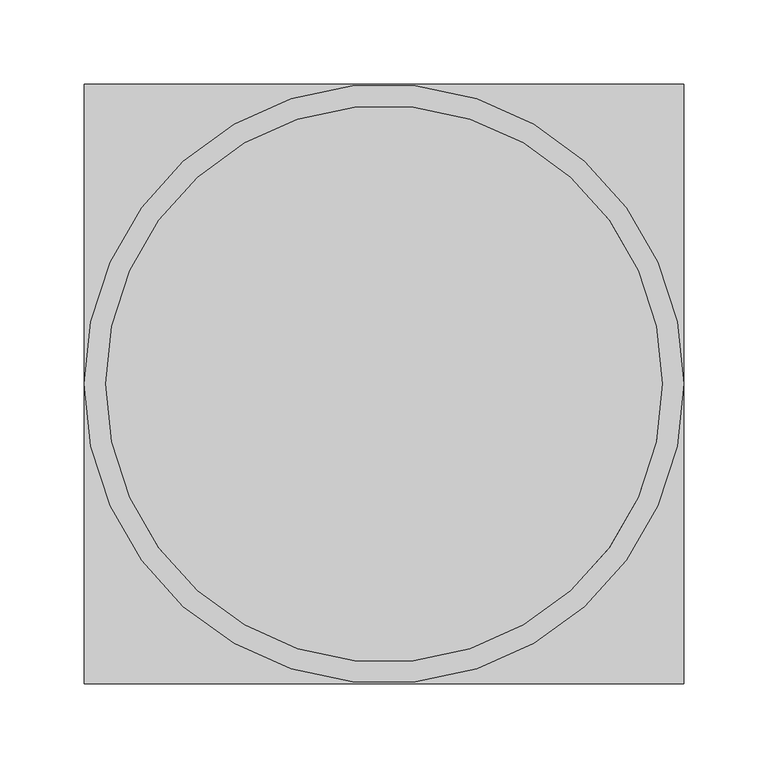
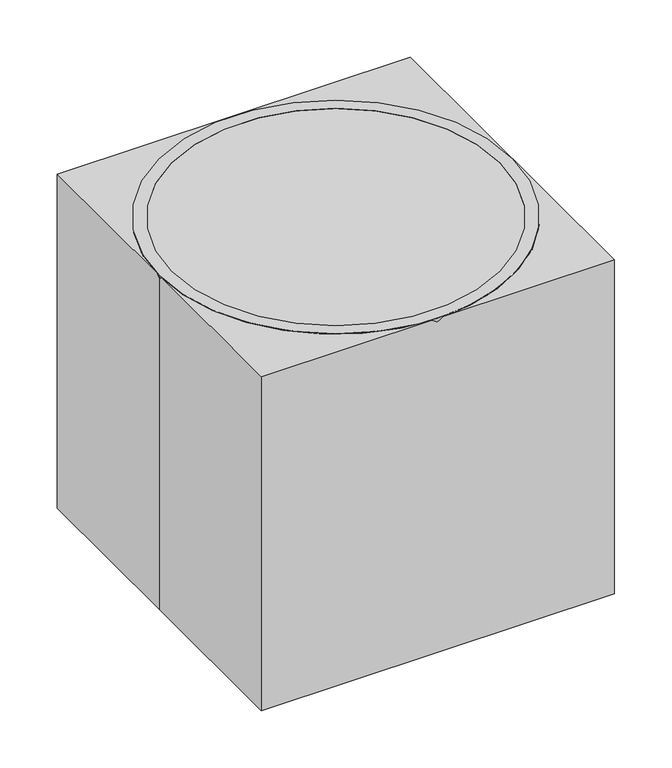
"""IFC4 building model written with IfcOpenShell, lengths in millimetres: proxy geometry, M8905 - Pail, Utility, CRS, Without Carriage : M8905 - Pail, Utility, CRS, Without Carriage."""

from ifc_helpers import new_model, si_unit, frame, origin, origin_with_axes, place, context, project, spatial, polyline, circle_curve, outline, extrude, source, transform, mapped, element, save
from ifc_brep_helpers import plane_surface, revolved_surface, advanced_brep


def specialty_equipment_c63f0c81(model_context):
    return source(origin(), model_context, "Body", "SolidModel", [
        advanced_brep(
        [(-127.0, 0.0, 0.0), (127.0, 0.0, 0.0), (-177.8, 0.0, 355.6), (177.8, 0.0, 355.6), (-165.1, 0.0, 355.6), (165.1, 0.0, 355.6), (114.3, 0.0, 19.5959229), (-114.3, 0.0, 19.5959229)],
        [
            (0, 1, circle_curve(frame((0.0, 0.0, 0.0), z_axis=(0.0, 0.0, -1.0), x_axis=(-1.0, 0.0, 0.0)), 127.0)),
            (1, 0, circle_curve(frame((0.0, 0.0, 0.0), z_axis=(0.0, 0.0, -1.0), x_axis=(1.0, 0.0, 0.0)), 127.0)),
            (2, 3, circle_curve(frame((0.0, 0.0, 355.6), z_axis=(0.0, 0.0, 1.0), x_axis=(1.0, 0.0, 0.0)), 177.8)),
            (3, 2, circle_curve(frame((0.0, 0.0, 355.6), z_axis=(0.0, 0.0, 1.0), x_axis=(-1.0, 0.0, 0.0)), 177.8)),
            (4, 5, circle_curve(frame((0.0, 0.0, 355.6), z_axis=(0.0, 0.0, -1.0), x_axis=(-1.0, 0.0, 0.0)), 165.1)),
            (5, 4, circle_curve(frame((0.0, 0.0, 355.6), z_axis=(0.0, 0.0, -1.0), x_axis=(1.0, 0.0, 0.0)), 165.1)),
            (1, 3),
            (2, 0),
            (6, 7, circle_curve(frame((0.0, 0.0, 19.5959229), z_axis=(0.0, 0.0, 1.0), x_axis=(-1.0, 0.0, 0.0)), 114.3)),
            (7, 6, circle_curve(frame((0.0, 0.0, 19.5959229), z_axis=(0.0, 0.0, 1.0), x_axis=(1.0, 0.0, 0.0)), 114.3)),
            (6, 5),
            (4, 7),
        ],
        [
            plane_surface(frame((0.0, 0.0, 0.0), z_axis=(0.0, 0.0, -1.0), x_axis=(0.0, -1.0, 0.0))),
            plane_surface(frame((0.0, 0.0, 355.6), z_axis=(0.0, 0.0, 1.0), x_axis=(0.0, -1.0, 0.0))),
            revolved_surface(polyline([(127.00000000000001, 0.0, 0.0), (177.8, 0.0, 355.5999999999999)]), (0.0, 0.0, -889.0), (0.0, 0.0, 1.0)),
            revolved_surface(polyline([(-127.00000000000001, 0.0, 0.0), (-177.8, 0.0, 355.5999999999999)]), (0.0, 0.0, -889.0), (0.0, 0.0, 1.0)),
            plane_surface(frame((0.0, 0.0, 19.5959229), z_axis=(0.0, 0.0, 1.0), x_axis=(0.0, -1.0, 0.0))),
            revolved_surface(polyline([(165.1, 0.0, 355.60000000000014), (114.299999996511, 0.0, 19.595922900000005)]), (0.0, 0.0, -736.4132505), (0.0, 0.0, 1.0)),
            revolved_surface(polyline([(-165.1, 0.0, 355.60000000000014), (-114.299999996511, 0.0, 19.595922900000005)]), (0.0, 0.0, -736.4132505), (0.0, 0.0, 1.0)),
        ],
        [
            (0, [[1, 2]]),
            (1, [[3, 4], [5, 6]]),
            (2, [[-2, 7, -3, 8]]),
            (3, [[-1, -8, -4, -7]]),
            (4, [[9, 10]]),
            (5, [[-9, 11, -5, 12]]),
            (6, [[-10, -12, -6, -11]]),
        ],
    ),
        extrude(outline(polyline([(-177.8, 177.8), (177.8, 177.8), (177.8, -177.8), (-177.8, -177.8), (-177.8, 0.0), (-177.8, 177.8)])), origin_with_axes(), (0.0, 0.0, 1.0), 355.6),
    ])


if __name__ == "__main__":
    model = new_model("IFC4")
    model_context = context("Model", 3, world=origin())
    ifc_project = project(units=[si_unit("LENGTHUNIT", "METRE", prefix="MILLI")], contexts=[model_context])
    site = spatial("IfcSite", under=ifc_project)
    building = spatial("IfcBuilding", under=site)
    placement = place(None, origin())
    specialty_equipment_shape = specialty_equipment_c63f0c81(model_context)
    element("IfcBuildingElementProxy", 1, Name="M8905 - Pail, Utility, CRS, Without Carriage : M8905 - Pail, Utility, CRS, Without Carriage", ObjectType="M8905 - Pail, Utility, CRS, Without Carriage : M8905 - Pail, Utility, CRS, Without Carriage", at=placement, inside=building, context=model_context, shape_type="MappedRepresentation", body=[
        mapped(specialty_equipment_shape, transform((0.0, 0.0, 0.0), x_axis=(1.0, 0.0, 0.0), y_axis=(0.0, 1.0, 0.0), z_axis=(0.0, 0.0, 1.0))),
    ])
    save(model, "model.ifc")

# Revit data of these elements
# Type "M8905 - Pail, Utility, CRS, Without Carriage : M8905 - Pail, Utility, CRS, Without Carriage"
#   Watts2 = "0"
#   Watts1 = "0"
#   Unit_Issue = "EA"
#   UTIL_6_Misc = "-"
#   UTIL_5_NonMedGas = "-"
#   UTIL_4_MiscGas = "-"
#   UTIL_3_MedGas = "-"
#   UTIL_2_Elec = "-"
#   UTIL_1_WaterDrain = "-"
#   Nomenclature = "Pail, Utility, CRS, Without Carriage"
#   NSN = "6530"
#   Location [instance default] = ""
#   JSN = "M8905"
#   Fund_Source_VA = "-"
#   Fund_Source_Navy = "-"
#   Fund_Source_Army = "-"
#   Fund_Source_AF = "-"
#   ELEC_Volts2 = "0"
#   ELEC_Volts1 = "0"
#   ELEC_Phase2 = "0"
#   ELEC_Phase1 = "0"
#   ELEC_HertzSwitch = "0"
#   ELEC_HertzDependent = "0"
#   ELEC_Hertz = "0"
#   ELEC_Amps2 = "0"
#   ELEC_Amps1 = "0"
#   DetailDescription = "Utility pail (kick bucket). Shall be a stainless steel 12 quart bucket for use in surgical operating rooms."
#   CAT_VA = "C"
#   CAT_Navy = "C"
#   CAT_IHS = "-"
#   CAT_Army = "C"
#   CAT_AF = "C"
#   BTUperhour = "0"
#   Weight_IP = 12
#   DIM_Width_IP = 1' - 2"
#   DIM_Height_IP = 1' - 2"
#   DIM_Depth_IP = 1' - 2"
#   finish [instance default] = none
# Element 1 (IfcBuildingElementProxy, "M8905 - Pail, Utility, CRS, Without Carriage : M8905 - Pail, Utility, CRS, Without Carriage")
#   Location = "ORGS1"
#   Materials on its faces: "EquipSpace"
# Materials
#   "EquipSpace": class "Unassigned", colour RGB 221 217 195, transparency 0.5
